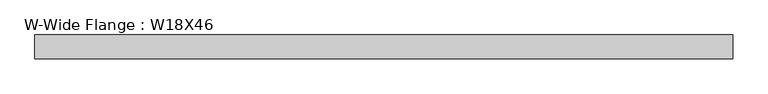
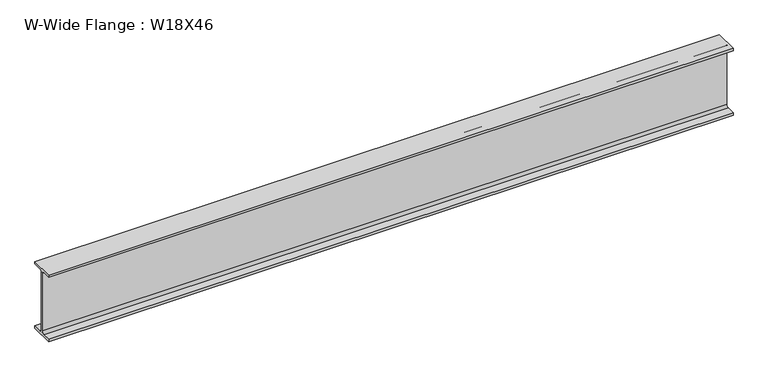
"""IFC4 building model written with IfcOpenShell, lengths in millimetres: beam geometry, W-Wide Flange : W18X46."""

from ifc_helpers import new_model, si_unit, point, frame, frame_2d, origin, place, context, project, spatial, polyline, circle_curve, trimmed, segment, composite_curve, outline, extrude, source, transform, mapped, element, save


def w_wide_flange_w18x46_e76c4543(model_context):
    return source(origin(), model_context, "Body", "SweptSolid", [
        extrude(outline(composite_curve([segment(polyline([(76.962, -214.503), (76.962, -229.87), (-76.962, -229.87), (-76.962, -214.503), (-20.955, -214.503)]), True, "CONTINUOUS"), segment(trimmed(circle_curve(frame_2d((-20.955, -198.12)), 16.383), [point((-20.955, -214.503))], [point((-4.572, -198.12))], True, "CARTESIAN"), True, "CONTINUOUS"), segment(polyline([(-4.572, -198.12), (-4.572, 198.12)]), True, "CONTINUOUS"), segment(trimmed(circle_curve(frame_2d((-20.955, 198.12)), 16.383), [point((-4.572, 198.12))], [point((-20.955, 214.503))], True, "CARTESIAN"), True, "CONTINUOUS"), segment(polyline([(-20.955, 214.503), (-76.962, 214.503), (-76.962, 229.87), (76.962, 229.87), (76.962, 214.503), (20.955, 214.503)]), True, "CONTINUOUS"), segment(trimmed(circle_curve(frame_2d((20.955, 198.12)), 16.383), [point((20.955, 214.503))], [point((4.572, 198.12))], True, "CARTESIAN"), True, "CONTINUOUS"), segment(polyline([(4.572, 198.12), (4.572, -198.12)]), True, "CONTINUOUS"), segment(trimmed(circle_curve(frame_2d((20.955, -198.12)), 16.383), [point((4.572, -198.12))], [point((20.955, -214.503))], True, "CARTESIAN"), True, "CONTINUOUS"), segment(polyline([(20.955, -214.503), (76.962, -214.503)]), True, "CONTINUOUS")], self_intersect=False)), frame((-2235.2, 0.0, 0.0), z_axis=(1.0, 0.0, 0.0), x_axis=(0.0, 1.0, 0.0)), (0.0, 0.0, 1.0), 4470.4),
    ])


if __name__ == "__main__":
    model = new_model("IFC4")
    model_context = context("Model", 3, world=origin())
    ifc_project = project(units=[si_unit("LENGTHUNIT", "METRE", prefix="MILLI")], contexts=[model_context])
    site = spatial("IfcSite", under=ifc_project)
    building = spatial("IfcBuilding", under=site)
    placement = place(None, origin())
    w_wide_flange_w18x46_shape = w_wide_flange_w18x46_e76c4543(model_context)
    element("IfcBeam", 1, ObjectType="W-Wide Flange : W18X46", at=placement, inside=building, context=model_context, shape_type="MappedRepresentation", body=[
        mapped(w_wide_flange_w18x46_shape, transform((0.0, 0.0, 0.0), x_axis=(1.0, 0.0, 0.0), y_axis=(0.0, 1.0, 0.0), z_axis=(0.0, 0.0, 1.0))),
    ])
    save(model, "model.ifc")

# Revit data of these elements
# Type "W-Wide Flange : W18X46"
#   Assembly Code = "B10"
#   W = 46
#   Length [instance default] = 5' - 0"
#   bf = 0' - 6.06"
#   d = 1' - 6.1"
#   k = 0' - 1 1/4"
#   k2 = 0' - 0.645"
#   tf = 0' - 0.605"
#   tw = 0' - 0.36"
#   A = 0.09375 SF
#   Structural Material [instance default] = Steel ASTM A992
# Element 1 (IfcBeam, "W-Wide Flange : W18X46")
#   Materials on its faces: "Steel ASTM A992"
# Materials
#   "Steel ASTM A992": class "Metal", colour RGB 199 199 199, transparency 0, Description = "Structural steel 50ksi", Cost = 0
